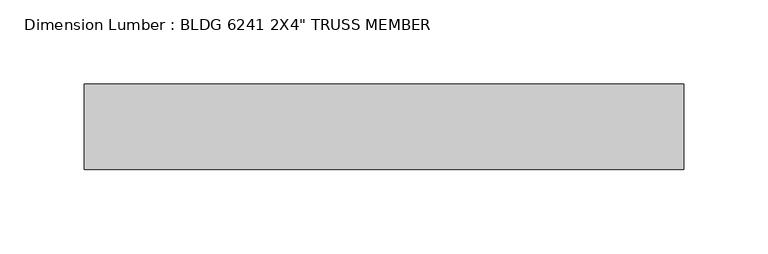
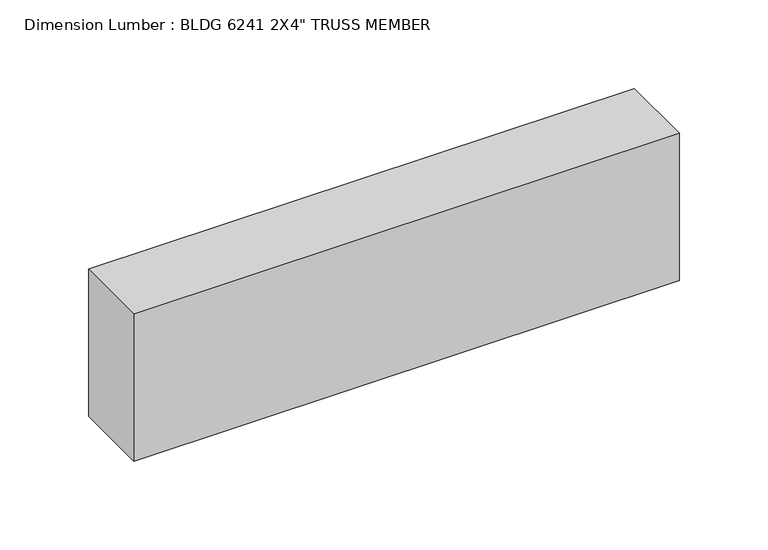
"""IFC4 building model written with IfcOpenShell, lengths in millimetres: beam geometry."""

from ifc_helpers import new_model, si_unit, frame, origin, place, context, project, spatial, polyline, outline, extrude, source, transform, mapped, element, save


def beam_90e8f76c(model_context):
    return source(origin(), model_context, "Body", "SweptSolid", [
        extrude(outline(polyline([(307.975, 25.4), (307.975, -25.4), (-47.625, -25.4), (-47.625, 25.4), (307.975, 25.4)])), frame((0.0, 0.0, -50.8), z_axis=(0.0, 0.0, 1.0), x_axis=(1.0, 0.0, 0.0)), (0.0, 0.0, 1.0), 101.6),
    ])


if __name__ == "__main__":
    model = new_model("IFC4")
    model_context = context("Model", 3, world=origin())
    ifc_project = project(units=[si_unit("LENGTHUNIT", "METRE", prefix="MILLI")], contexts=[model_context])
    site = spatial("IfcSite", under=ifc_project)
    building = spatial("IfcBuilding", under=site)
    placement = place(None, origin())
    beam_shape = beam_90e8f76c(model_context)
    element("IfcBeam", 1, ObjectType="Dimension Lumber : BLDG 6241 2X4\" TRUSS MEMBER", at=placement, inside=building, context=model_context, shape_type="MappedRepresentation", body=[
        mapped(beam_shape, transform((0.0, 0.0, 0.0), x_axis=(1.0, 0.0, 0.0), y_axis=(0.0, 1.0, 0.0), z_axis=(0.0, 0.0, 1.0))),
    ])
    save(model, "model.ifc")

# Revit data of these elements
# Type "Dimension Lumber : BLDG 6241 2X4\" TRUSS MEMBER"
#   Assembly Code = "B10"
#   A = 0.273472 SF
#   Length [instance default] = 5' - 0"
#   b = 0' - 2"
#   d = 0' - 4"
#   Structural Material [instance default] = Softwood, Lumber
# Element 1 (IfcBeam, "Dimension Lumber : BLDG 6241 2X4\" TRUSS MEMBER")
#   Materials on its faces: "Softwood, Lumber"
# Materials
#   "Softwood, Lumber": class "Wood", colour RGB 223 192 134, transparency 0, Description = "Pinus Echinata", Cost = 0
